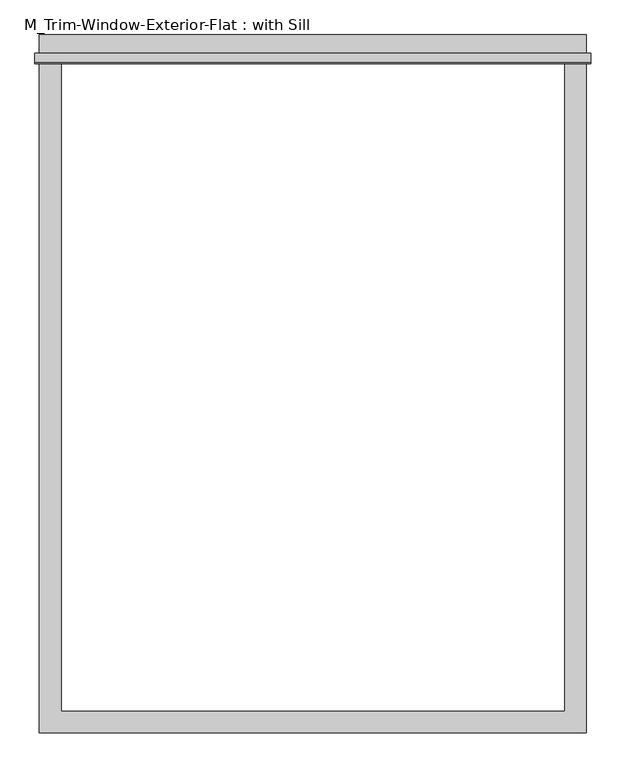
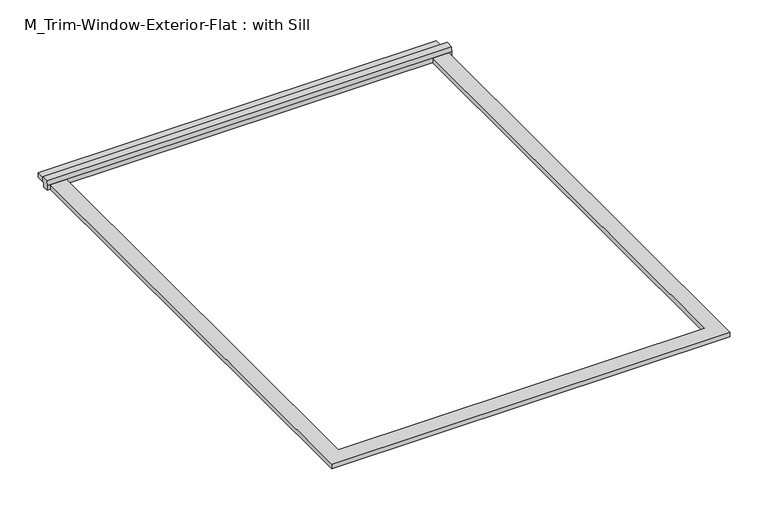
"""IFC4 building model written with IfcOpenShell, lengths in millimetres: proxy geometry, M_Trim-Window-Exterior-Flat : with Sill."""

from ifc_helpers import new_model, si_unit, frame, origin, origin_with_axes, place, context, project, spatial, polyline, outline, extrude, source, transform, mapped, element, save


def m_trim_window_exterior_flat_with_sill_88aaac3a(model_context):
    return source(origin(), model_context, "Body", "SweptSolid", [
        extrude(outline(polyline([(760.0, 1820.4323709), (-760.0, 1820.4323709), (-760.0, 1880.4323709), (760.0, 1880.4323709), (760.0, 1820.4323709)])), origin_with_axes(), (0.0, 0.0, 1.0), 19.05),
        extrude(outline(polyline([(1830.0, 38.1), (1830.0, 19.05), (1820.4323709, 19.05), (1820.4323709, 0.0), (1800.0, 0.0), (1800.0, 19.05), (1802.4580645, 38.1), (1830.0, 38.1)])), frame((-772.7, 0.0, 0.0), z_axis=(1.0, 0.0, 0.0), x_axis=(0.0, 1.0, 0.0)), (0.0, 0.0, 1.0), 1545.4),
        extrude(outline(polyline([(-760.0, -60.0), (-760.0, 1800.0), (-700.0, 1800.0), (-700.0, 0.0), (700.0, 0.0), (700.0, 1800.0), (760.0, 1800.0), (760.0, -60.0), (-760.0, -60.0)])), origin_with_axes(), (0.0, 0.0, 1.0), 19.05),
    ])


if __name__ == "__main__":
    model = new_model("IFC4")
    model_context = context("Model", 3, world=origin())
    ifc_project = project(units=[si_unit("LENGTHUNIT", "METRE", prefix="MILLI")], contexts=[model_context])
    site = spatial("IfcSite", under=ifc_project)
    building = spatial("IfcBuilding", under=site)
    placement = place(None, origin())
    m_trim_window_exterior_flat_with_sill_shape = m_trim_window_exterior_flat_with_sill_88aaac3a(model_context)
    element("IfcBuildingElementProxy", 1, Name="M_Trim-Window-Exterior-Flat : with Sill", ObjectType="M_Trim-Window-Exterior-Flat : with Sill", at=placement, inside=building, context=model_context, shape_type="MappedRepresentation", body=[
        mapped(m_trim_window_exterior_flat_with_sill_shape, transform((0.0, 0.0, 0.0), x_axis=(1.0, 0.0, 0.0), y_axis=(0.0, 1.0, 0.0), z_axis=(0.0, 0.0, 1.0))),
    ])
    save(model, "model.ifc")

# Revit data of these elements
# Type "M_Trim-Window-Exterior-Flat : with Sill"
#   Trim Width = 60 mm
#   Trim Thickness_Picture Frame = 30 mm
#   Trim Thickness_with Sill = 19.05 mm
#   Sill Thickness = 30 mm
#   Opening Width [instance default] = 600 mm
#   Opening Height [instance default] = 900 mm
#   Default Elevation = 1200 mm
#   Sill = yes
#   Picture Frame = no
#   Trim Material [instance default] = none
# Element 1 (IfcBuildingElementProxy, "M_Trim-Window-Exterior-Flat : with Sill")
#   Opening Width = 1400 mm
#   Opening Height = 1800 mm
#   Trim Material = Clad - White
#   Materials on its faces: "Clad - White"
# Materials
#   "Clad - White": class "Wood", colour RGB 245 245 243, transparency 0, Cost = 0
